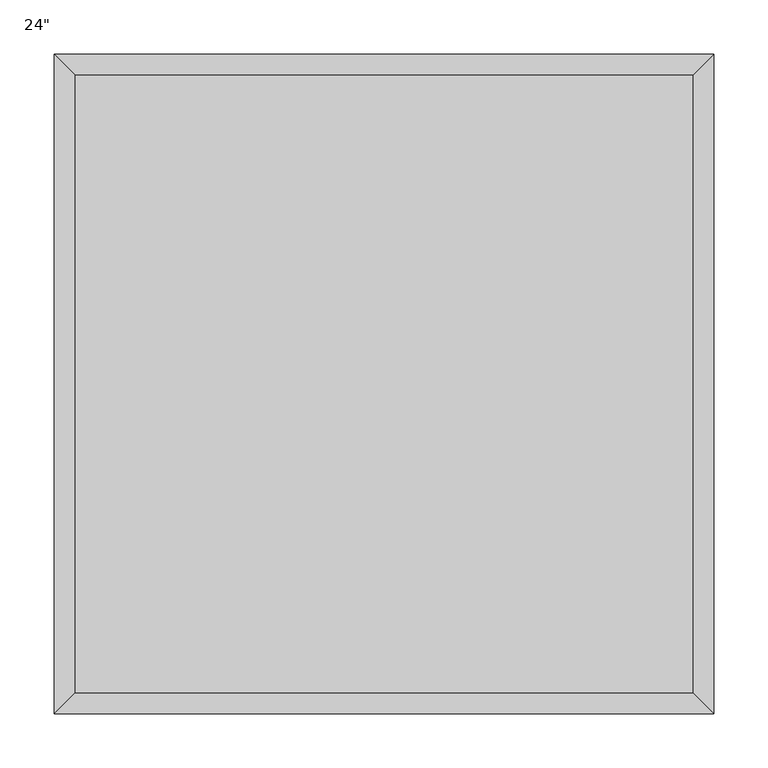
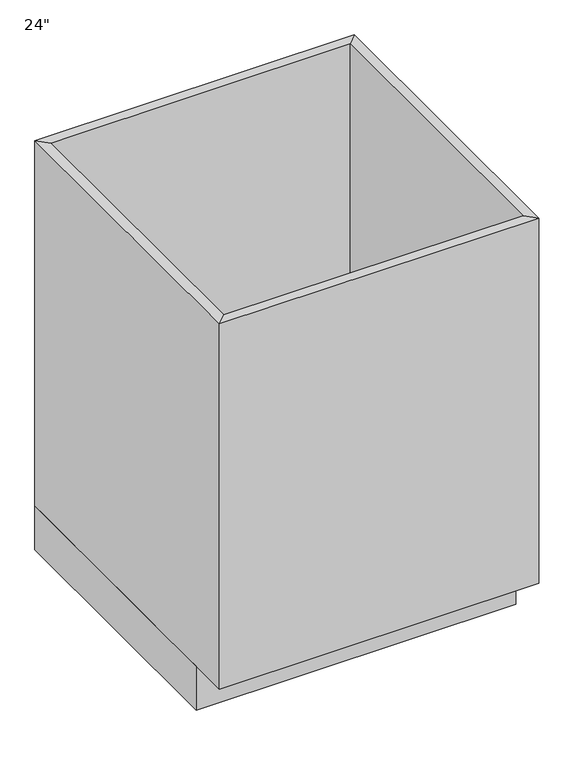
"""IFC4 building model written with IfcOpenShell, lengths in millimetres: furniture geometry."""

import ifcopenshell
import ifcopenshell.guid

model = None  # the IFC model being written
_history = None  # IfcOwnerHistory: only IFC2X3 demands one
_inside = {}  # id of a spatial element -> (the spatial element, [elements in it])
_under = {}  # id of a project, library or spatial element -> (it, [spatial elements below it])
_declared = {}  # id of a project -> (the project, [libraries it declares])
_typed = {}  # id of a type object -> (the type object, [elements of that type])
_made_of = {}  # id of a material, layer set ... -> (it, [elements and type objects made of it])


def new_model(schema):
    """Start an empty IFC model of exactly this schema.

    Asked for "IFC4X3", IfcOpenShell would pick the latest addendum, in which some entities
    have other attributes; the version numbers below select the first issue.
    IFC2X3 requires an IfcOwnerHistory on every rooted entity: one is made here for all.
    """
    global model, _history
    if schema == "IFC4X3":
        model = ifcopenshell.file(schema_version=(4, 3, 0, 0))
    else:
        model = ifcopenshell.file(schema=schema)
    _inside.clear()
    _under.clear()
    _declared.clear()
    _typed.clear()
    _made_of.clear()
    _history = None
    if model.schema == "IFC2X3":
        org = make("IfcOrganization", Name="unknown")
        user = make(
            "IfcPersonAndOrganization",
            ThePerson=make("IfcPerson", FamilyName="unknown"),
            TheOrganization=org,
        )
        app = make(
            "IfcApplication",
            ApplicationDeveloper=org,
            Version="unknown",
            ApplicationFullName="unknown",
            ApplicationIdentifier="unknown",
        )
        _history = make(
            "IfcOwnerHistory",
            OwningUser=user,
            OwningApplication=app,
            ChangeAction="ADDED",
            CreationDate=0,
        )
    return model


def make(cls, **values):
    """One entity of the class cls with the attributes given. An attribute that is None is left unset."""
    return model.create_entity(
        cls, **{name: value for name, value in values.items() if value is not None}
    )


def rooted(cls, **values):
    """An entity with a GlobalId (a new one), such as an element, a storey or a relation."""
    return make(cls, GlobalId=ifcopenshell.guid.new(), OwnerHistory=_history, **values)


def si_unit(unit_type, name, prefix=None):
    """IfcSIUnit, for example si_unit("LENGTHUNIT", "METRE", prefix="MILLI")."""
    return make("IfcSIUnit", UnitType=unit_type, Prefix=prefix, Name=name)


def assignment(units):
    """IfcUnitAssignment: the units of a project."""
    return None if units is None else make("IfcUnitAssignment", Units=units)


def point(xyz):
    """IfcCartesianPoint."""
    return None if xyz is None else make("IfcCartesianPoint", Coordinates=xyz)


def direction(xyz):
    """IfcDirection."""
    return None if xyz is None else make("IfcDirection", DirectionRatios=xyz)


def frame(location, z_axis=None, x_axis=None):
    """IfcAxis2Placement3D, a coordinate frame: its origin and axes. An axis left out is left unset."""
    return make(
        "IfcAxis2Placement3D",
        Location=point(location),
        Axis=direction(z_axis),
        RefDirection=direction(x_axis),
    )


def origin():
    """The frame at (0, 0, 0) with its axes left unset."""
    return frame((0.0, 0.0, 0.0))


def origin_with_axes():
    """The frame at (0, 0, 0) with the z axis (0, 0, 1) and the x axis (1, 0, 0) written out."""
    return frame((0.0, 0.0, 0.0), z_axis=(0.0, 0.0, 1.0), x_axis=(1.0, 0.0, 0.0))


def place(relative_to, where):
    """IfcLocalPlacement: puts the frame where relative to a parent placement (None: the world)."""
    return make(
        "IfcLocalPlacement", PlacementRelTo=relative_to, RelativePlacement=where
    )


def context(
    kind, dimensions, precision=None, world=None, true_north=None, identifier=None
):
    """IfcGeometricRepresentationContext, for example the 3D "Model" context."""
    return make(
        "IfcGeometricRepresentationContext",
        ContextIdentifier=identifier,
        ContextType=kind,
        CoordinateSpaceDimension=dimensions,
        Precision=precision,
        WorldCoordinateSystem=world,
        TrueNorth=true_north,
    )


def project(units=None, contexts=None):
    """IfcProject with its units and contexts."""
    return rooted(
        "IfcProject",
        Name="project",
        RepresentationContexts=contexts,
        UnitsInContext=assignment(units),
    )


def spatial(cls, under=None, at=None, **own):
    """A site, building, storey or space (cls), placed at a placement, below another one or the project."""
    s = rooted(cls, ObjectPlacement=at, **own)
    if under is not None:
        _under.setdefault(under.id(), (under, []))[1].append(s)
    return s


def polyline(points):
    """IfcPolyline through the points."""
    return make("IfcPolyline", Points=[point(p) for p in points])


def outline(outer, holes=None, kind="AREA"):
    """IfcArbitraryClosedProfileDef: a profile drawn as a closed curve; with holes, ...WithVoids."""
    if holes is None:
        return make("IfcArbitraryClosedProfileDef", ProfileType=kind, OuterCurve=outer)
    return make(
        "IfcArbitraryProfileDefWithVoids",
        ProfileType=kind,
        OuterCurve=outer,
        InnerCurves=holes,
    )


def extrude(swept, where, along, depth):
    """IfcExtrudedAreaSolid: the profile swept, set in the frame where, extruded along a direction by depth."""
    return make(
        "IfcExtrudedAreaSolid",
        SweptArea=swept,
        Position=where,
        ExtrudedDirection=direction(along),
        Depth=depth,
    )


def faces_of(points, faces, orient=None, outer=None):
    """IfcFace entities. A face is a list of loops; a loop is a list of indices into points, from 0.

    orient and outer hold one flag for each loop. By default every Orientation is true, the
    first loop of a face is its IfcFaceOuterBound and the others are IfcFaceBound.
    """
    made = []
    for i, loops in enumerate(faces):
        bounds = []
        for j, loop in enumerate(loops):
            is_outer = j == 0 if outer is None else outer[i][j]
            bounds.append(
                make(
                    "IfcFaceOuterBound" if is_outer else "IfcFaceBound",
                    Bound=make("IfcPolyLoop", Polygon=[points[k] for k in loop]),
                    Orientation=True if orient is None else orient[i][j],
                )
            )
        made.append(make("IfcFace", Bounds=bounds))
    return made


def faceted_brep(points, faces, orient=None, outer=None, voids=None):
    """IfcFacetedBrep: a solid bounded by flat faces; with voids (closed shells), ...WithVoids."""
    shared = [point(p) for p in points]
    hull = make("IfcClosedShell", CfsFaces=faces_of(shared, faces, orient, outer))
    if voids is None:
        return make("IfcFacetedBrep", Outer=hull)
    return make(
        "IfcFacetedBrepWithVoids",
        Outer=hull,
        Voids=[
            make(cls, CfsFaces=faces_of(shared, fs, o, b)) for cls, fs, o, b in voids
        ],
    )


def shape(context_of_items, identifier, shape_type, items):
    """IfcShapeRepresentation: the items that make up one representation, for example the "Body"."""
    return make(
        "IfcShapeRepresentation",
        ContextOfItems=context_of_items,
        RepresentationIdentifier=identifier,
        RepresentationType=shape_type,
        Items=items,
    )


def source(mapping_origin, context_of_items, identifier, shape_type, items):
    """IfcRepresentationMap: a shape defined once, which mapped items show again and again."""
    return make(
        "IfcRepresentationMap",
        MappingOrigin=mapping_origin,
        MappedRepresentation=shape(context_of_items, identifier, shape_type, items),
    )


def transform(
    local_origin,
    x_axis=None,
    y_axis=None,
    z_axis=None,
    scale=None,
    scale2=None,
    scale3=None,
    uniform=True,
):
    """IfcCartesianTransformationOperator3D, or its non-uniform kind. x_axis, y_axis, z_axis: its Axis1, 2, 3."""
    if uniform:
        return make(
            "IfcCartesianTransformationOperator3D",
            Axis1=direction(x_axis),
            Axis2=direction(y_axis),
            LocalOrigin=point(local_origin),
            Scale=scale,
            Axis3=direction(z_axis),
        )
    return make(
        "IfcCartesianTransformationOperator3DnonUniform",
        Axis1=direction(x_axis),
        Axis2=direction(y_axis),
        LocalOrigin=point(local_origin),
        Scale=scale,
        Axis3=direction(z_axis),
        Scale2=scale2,
        Scale3=scale3,
    )


def mapped(mapping_source, mapping_target):
    """IfcMappedItem: shows the shape of a source again, moved by a transform."""
    return make(
        "IfcMappedItem", MappingSource=mapping_source, MappingTarget=mapping_target
    )


def made_of(thing, what):
    """Note that an element or type object is made of a material, layer set ...; save() writes the relation."""
    if what is not None:
        _made_of.setdefault(what.id(), (what, []))[1].append(thing)
    return thing


def element(
    cls,
    number,
    at=None,
    inside=None,
    cuts=None,
    type_object=None,
    material=None,
    context=None,
    identifier="Body",
    shape_type=None,
    held_by="IfcProductDefinitionShape",
    body=None,
    shapes=None,
    **own,
):
    """One element of the class cls, such as IfcWall. Its Tag is "e" and its number.

    at: its placement. inside: the storey or other place that contains it. cuts: it is an
    opening in that element (IfcRelVoidsElement). A single representation is given by context,
    identifier, shape_type and body (its items); several are given by shapes. held_by: the class
    of the entity that holds the representations. save() writes the other relations.
    """
    e = rooted(cls, Tag="e%d" % number, ObjectPlacement=at, **own)
    if body is not None:
        shapes = [shape(context, identifier, shape_type, body)]
    if shapes is not None:
        e.Representation = make(held_by, Representations=shapes)
    if inside is not None:
        _inside.setdefault(inside.id(), (inside, []))[1].append(e)
    if cuts is not None:
        rooted(
            "IfcRelVoidsElement", RelatingBuildingElement=cuts, RelatedOpeningElement=e
        )
    if type_object is not None:
        _typed.setdefault(type_object.id(), (type_object, []))[1].append(e)
    return made_of(e, material)


def aggregate(whole, parts):
    """IfcRelAggregates: a whole, such as a stair, and the parts it consists of."""
    return rooted("IfcRelAggregates", RelatingObject=whole, RelatedObjects=parts)


def save(model, path):
    """Write the relations noted so far, then the file.

    IfcRelAggregates (storeys below a building ...), IfcRelContainedInSpatialStructure (elements
    in a storey), IfcRelDefinesByType, IfcRelAssociatesMaterial and IfcRelDeclares: one each for
    every whole, place, type object, material and project.
    """
    for whole, parts in _under.values():
        aggregate(whole, parts)
    for where, things in _inside.values():
        rooted(
            "IfcRelContainedInSpatialStructure",
            RelatedElements=things,
            RelatingStructure=where,
        )
    for kind, things in _typed.values():
        rooted("IfcRelDefinesByType", RelatedObjects=things, RelatingType=kind)
    for what, things in _made_of.values():
        rooted("IfcRelAssociatesMaterial", RelatedObjects=things, RelatingMaterial=what)
    for by, libraries in _declared.values():
        rooted("IfcRelDeclares", RelatingContext=by, RelatedDefinitions=libraries)
    model.write(path)


def furniture_31151d79(model_context):
    return source(origin(), model_context, "Body", "SolidModel", [
        extrude(outline(polyline([(304.4877049, -19.05), (304.4877049, -590.55), (-267.0122951, -590.55), (-267.0122951, -19.05), (304.4877049, -19.05)])), frame((0.0, 0.0, 88.9), z_axis=(0.0, 0.0, 1.0), x_axis=(1.0, 0.0, 0.0)), (0.0, 0.0, 1.0), 19.05),
        faceted_brep([(304.4877049, -590.55, 825.5), (304.4877049, -590.55, 88.9), (-267.0122951, -590.55, 88.9), (-267.0122951, -590.55, 825.5), (323.5377049, -609.6, 825.5), (-286.0622951, -609.6, 825.5), (323.5377049, -609.6, 88.9), (-286.0622951, -609.6, 88.9), (-267.0122951, -19.05, 88.9), (-267.0122951, -19.05, 825.5), (-286.0622951, 0.0, 825.5), (-286.0622951, 0.0, 88.9), (304.4877049, -19.05, 88.9), (304.4877049, -19.05, 825.5), (323.5377049, 0.0, 825.5), (323.5377049, 0.0, 88.9)], [[[0, 1, 2, 3]], [[4, 0, 3, 5]], [[6, 4, 5, 7]], [[1, 6, 7, 2]], [[3, 2, 8, 9]], [[5, 3, 9, 10]], [[7, 5, 10, 11]], [[2, 7, 11, 8]], [[9, 8, 12, 13]], [[10, 9, 13, 14]], [[11, 10, 14, 15]], [[8, 11, 15, 12]], [[13, 12, 1, 0]], [[14, 13, 0, 4]], [[15, 14, 4, 6]], [[12, 15, 6, 1]]]),
        extrude(outline(polyline([(323.5377049, 0.0), (323.5377049, -533.4), (-286.0622951, -533.4), (-286.0622951, 0.0), (323.5377049, 0.0)])), origin_with_axes(), (0.0, 0.0, 1.0), 88.9),
    ])


if __name__ == "__main__":
    model = new_model("IFC4")
    model_context = context("Model", 3, world=origin())
    ifc_project = project(units=[si_unit("LENGTHUNIT", "METRE", prefix="MILLI")], contexts=[model_context])
    site = spatial("IfcSite", under=ifc_project)
    building = spatial("IfcBuilding", under=site)
    placement = place(None, origin())
    furniture_shape = furniture_31151d79(model_context)
    element("IfcFurniture", 1, ObjectType="Base Cabinet-Single Door & Drawer : 24\"", at=placement, inside=building, context=model_context, shape_type="MappedRepresentation", body=[
        mapped(furniture_shape, transform((0.0, 0.0, 0.0), x_axis=(1.0, 0.0, 0.0), y_axis=(0.0, 1.0, 0.0), z_axis=(0.0, 0.0, 1.0))),
    ])
    save(model, "model.ifc")

# Revit data of these elements
# Type "Base Cabinet-Single Door & Drawer : 24\""
#   Depth = 2' - 0"
#   Height = 2' - 8 1/2"
#   Toe Depth = 0' - 3"
#   Toe Height = 0' - 3 1/2"
#   Width = 2' - 0"
# Element 1 (IfcFurniture, "Base Cabinet-Single Door & Drawer : 24\"")
#   Materials on its faces: "CASEWORK"
# Materials
#   "CASEWORK": class "Generic", colour RGB 181 181 181, transparency 0, Cost = 0
